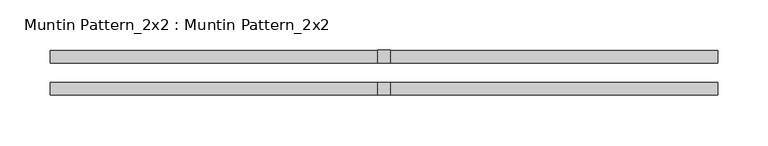
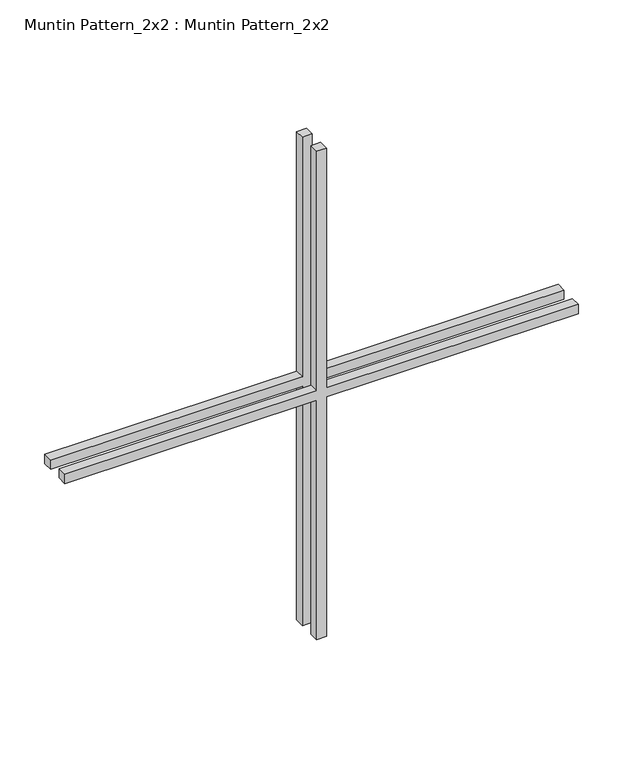
"""IFC4 building model written with IfcOpenShell, lengths in millimetres: proxy geometry, Muntin Pattern_2x2 : Muntin Pattern_2x2."""

from ifc_helpers import new_model, si_unit, frame, origin, place, context, project, spatial, polyline, outline, extrude, source, transform, mapped, element, save


def muntin_pattern_2x2_muntin_pattern_2x2_7e768004(model_context):
    return source(origin(), model_context, "Body", "SweptSolid", [
        extrude(outline(polyline([(338.1375, -6.35), (338.1375, -330.2), (325.4375, -330.2), (325.4375, -6.35), (0.0, -6.35), (0.0, 6.35), (325.4375, 6.35), (325.4375, 330.2), (338.1375, 330.2), (338.1375, 6.35), (663.575, 6.35), (663.575, -6.35), (338.1375, -6.35)])), frame((0.0, -22.225, 0.0), z_axis=(0.0, 1.0, 0.0), x_axis=(0.0, 0.0, 1.0)), (0.0, 0.0, 1.0), 12.7),
        extrude(outline(polyline([(338.1375, -6.35), (338.1375, -330.2), (325.4375, -330.2), (325.4375, -6.35), (0.0, -6.35), (0.0, 6.35), (325.4375, 6.35), (325.4375, 330.2), (338.1375, 330.2), (338.1375, 6.35), (663.575, 6.35), (663.575, -6.35), (338.1375, -6.35)])), frame((0.0, 9.525, 0.0), z_axis=(0.0, 1.0, 0.0), x_axis=(0.0, 0.0, 1.0)), (0.0, 0.0, 1.0), 12.7),
    ])


if __name__ == "__main__":
    model = new_model("IFC4")
    model_context = context("Model", 3, world=origin())
    ifc_project = project(units=[si_unit("LENGTHUNIT", "METRE", prefix="MILLI")], contexts=[model_context])
    site = spatial("IfcSite", under=ifc_project)
    building = spatial("IfcBuilding", under=site)
    placement = place(None, origin())
    muntin_pattern_2x2_muntin_pattern_2x2_shape = muntin_pattern_2x2_muntin_pattern_2x2_7e768004(model_context)
    element("IfcBuildingElementProxy", 1, Name="Muntin Pattern_2x2 : Muntin Pattern_2x2", ObjectType="Muntin Pattern_2x2 : Muntin Pattern_2x2", at=placement, inside=building, context=model_context, shape_type="MappedRepresentation", body=[
        mapped(muntin_pattern_2x2_muntin_pattern_2x2_shape, transform((0.0, 0.0, 0.0), x_axis=(1.0, 0.0, 0.0), y_axis=(0.0, 1.0, 0.0), z_axis=(0.0, 0.0, 1.0))),
    ])
    save(model, "model.ifc")

# Revit data of these elements
# Type "Muntin Pattern_2x2 : Muntin Pattern_2x2"
#   Width [instance default] = 4' - 0"
#   Thickness = 0' - 0 1/2"
#   Height [instance default] = 4' - 0"
#   Distance = 0' - 0 3/4"
#   Interior Material [instance default] = none
#   Exterior Material [instance default] = none
#   Default Elevation = 0
# Element 1 (IfcBuildingElementProxy, "Muntin Pattern_2x2 : Muntin Pattern_2x2")
#   Width = 2' - 2"
#   Height = 2' - 2 1/8"
#   Interior Material = Wood - Stained
#   Exterior Material = Clad - White
#   Materials on its faces: "Clad - White", "Wood - Stained"
# Materials
#   "Clad - White": class "Wood", colour RGB 242 242 238, transparency 0, Cost = 0
#   "Wood - Stained": class "Wood", colour RGB 224 178 126, transparency 0, Cost = 0
